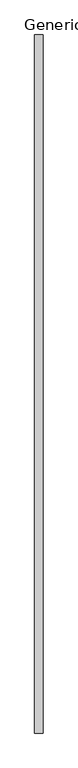
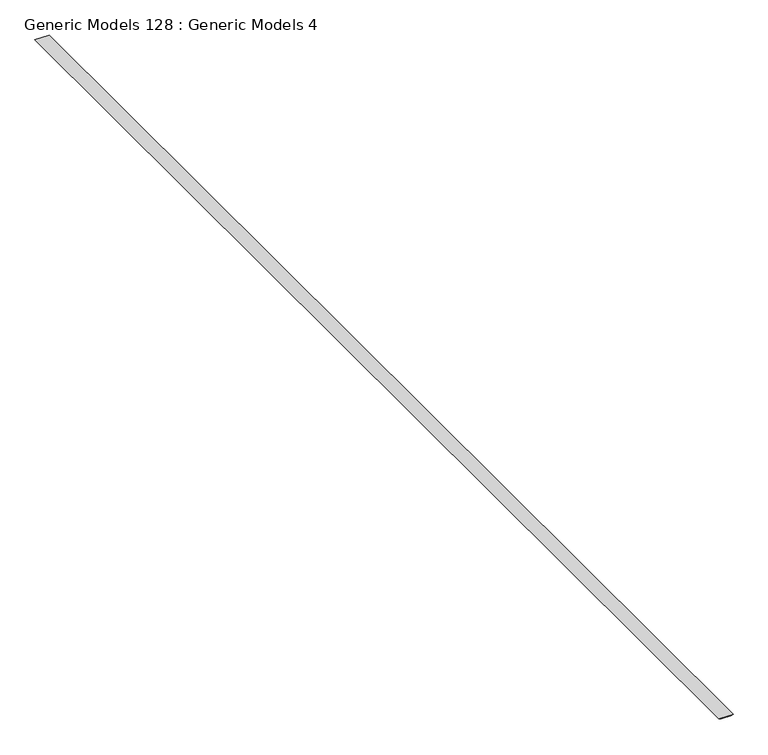
"""IFC4 building model written with IfcOpenShell, lengths in millimetres: proxy geometry, Generic Models 128 : Generic Models 4."""

from ifc_helpers import new_model, si_unit, frame, origin, place, context, project, spatial, polyline, outline, extrude, source, transform, mapped, element, save


def generic_models_128_generic_models_4_4ec3f272(model_context):
    return source(origin(), model_context, "Body", "SweptSolid", [
        extrude(outline(polyline([(127085.980596, 7267.0334328), (127103.0817625, 7300.3357046), (127107.6883511, 7075.5816217), (127089.1652967, 7111.6528329), (127085.980596, 7267.0334328)])), frame((0.0, -6864.9230338, 0.0), z_axis=(0.0, 1.0, 0.0), x_axis=(0.0, 0.0, 1.0)), (0.0, 0.0, 1.0), 18643.6),
    ])


if __name__ == "__main__":
    model = new_model("IFC4")
    model_context = context("Model", 3, world=origin())
    ifc_project = project(units=[si_unit("LENGTHUNIT", "METRE", prefix="MILLI")], contexts=[model_context])
    site = spatial("IfcSite", under=ifc_project)
    building = spatial("IfcBuilding", under=site)
    placement = place(None, origin())
    generic_models_128_generic_models_4_shape = generic_models_128_generic_models_4_4ec3f272(model_context)
    element("IfcBuildingElementProxy", 1, Name="Generic Models 128 : Generic Models 4", ObjectType="Generic Models 128 : Generic Models 4", at=placement, inside=building, context=model_context, shape_type="MappedRepresentation", body=[
        mapped(generic_models_128_generic_models_4_shape, transform((0.0, 0.0, 0.0), x_axis=(1.0, 0.0, 0.0), y_axis=(0.0, 1.0, 0.0), z_axis=(0.0, 0.0, 1.0))),
    ])
    save(model, "model.ifc")

# Revit data of these elements
# Element 1 (IfcBuildingElementProxy, "Generic Models 128 : Generic Models 4")
#   Materials on its faces: "_7/8\" SMOOTH TROWEL EXTERIOR STUCCO (COLOR PER OWNER) @ 2% SLOPE"
# Materials
#   "_7/8\" SMOOTH TROWEL EXTERIOR STUCCO (COLOR PER OWNER) @ 2% SLOPE": class "Generic", colour RGB 233 233 233, transparency 0, Cost = 0
